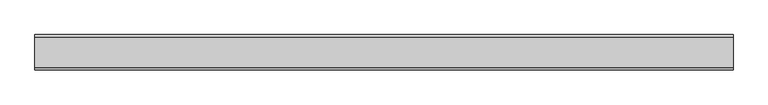
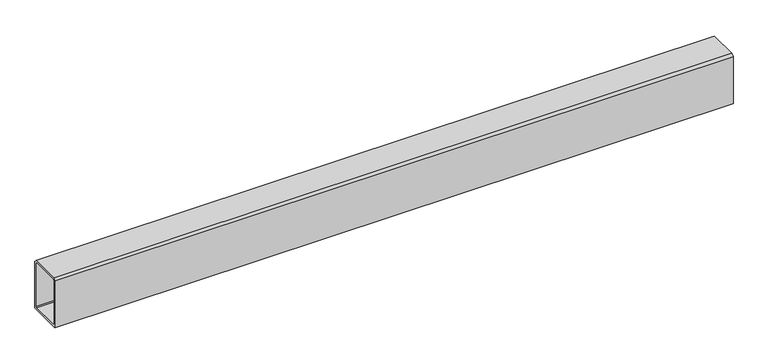
"""IFC4 building model written with IfcOpenShell, lengths in millimetres: proxy geometry, Door frame3:Door frame019:291314 : Door frame3:Door frame019:291314."""

from ifc_helpers import new_model, si_unit, frame, origin, place, context, project, spatial, polyline, outline, extrude, source, transform, mapped, element, save


def generic_models_d94b4cc0(model_context):
    return source(origin(), model_context, "Body", "SweptSolid", [
        extrude(outline(polyline([(9929.1876525, 39484.0466875), (10018.0876525, 39484.0466875), (10024.4376525, 39477.6966875), (10024.4376525, 39331.6466875), (9922.8376525, 39331.6466875), (9922.8376525, 39477.6966875), (9929.1876525, 39484.0466875)]), holes=[polyline([(10015.4573964, 39337.9966875), (10018.0876525, 39340.6269436), (10018.0876525, 39475.0664314), (10015.4573964, 39477.6966875), (9931.8179086, 39477.6966875), (9929.1876525, 39475.0664314), (9929.1876525, 39340.6269436), (9931.8179086, 39337.9966875), (10015.4573964, 39337.9966875)])]), frame((-4455.0628198, 0.0, 0.0), z_axis=(1.0, 0.0, 0.0), x_axis=(0.0, 1.0, 0.0)), (0.0, 0.0, 1.0), 1999.85),
    ])


if __name__ == "__main__":
    model = new_model("IFC4")
    model_context = context("Model", 3, world=origin())
    ifc_project = project(units=[si_unit("LENGTHUNIT", "METRE", prefix="MILLI")], contexts=[model_context])
    site = spatial("IfcSite", under=ifc_project)
    building = spatial("IfcBuilding", under=site)
    placement = place(None, origin())
    generic_models_shape = generic_models_d94b4cc0(model_context)
    element("IfcBuildingElementProxy", 1, Name="Door frame3:Door frame019:291314 : Door frame3:Door frame019:291314", ObjectType="Door frame3:Door frame019:291314 : Door frame3:Door frame019:291314", at=placement, inside=building, context=model_context, shape_type="MappedRepresentation", body=[
        mapped(generic_models_shape, transform((0.0, 0.0, 0.0), x_axis=(1.0, 0.0, 0.0), y_axis=(0.0, 1.0, 0.0), z_axis=(0.0, 0.0, 1.0))),
    ])
    save(model, "model.ifc")

# Revit data of these elements
# Type "Door frame3:Door frame019:291314 : Door frame3:Door frame019:291314"
#   NameOverride = "Door frame3:Door frame019:291314"
#   ObjectTypeOverride = "Door frame3:Door frame019"
#   Reference = "Door frame019"
#   Category = "Generic Models"
#   Tag = "291314"
# Element 1 (IfcBuildingElementProxy, "Door frame3:Door frame019:291314 : Door frame3:Door frame019:291314")
#   Materials on its faces: "TUBE STEEL PROFILE - METALIZED, PRIMED & PAINTED (COLOR PER ARCHITECT)"
# Materials
#   "TUBE STEEL PROFILE - METALIZED, PRIMED & PAINTED (COLOR PER ARCHITECT)": class "Unassigned", colour RGB 128 128 128, transparency 0
